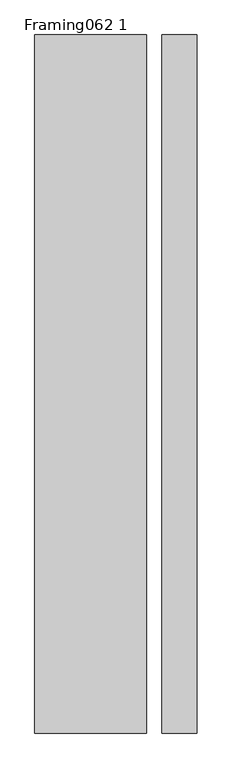
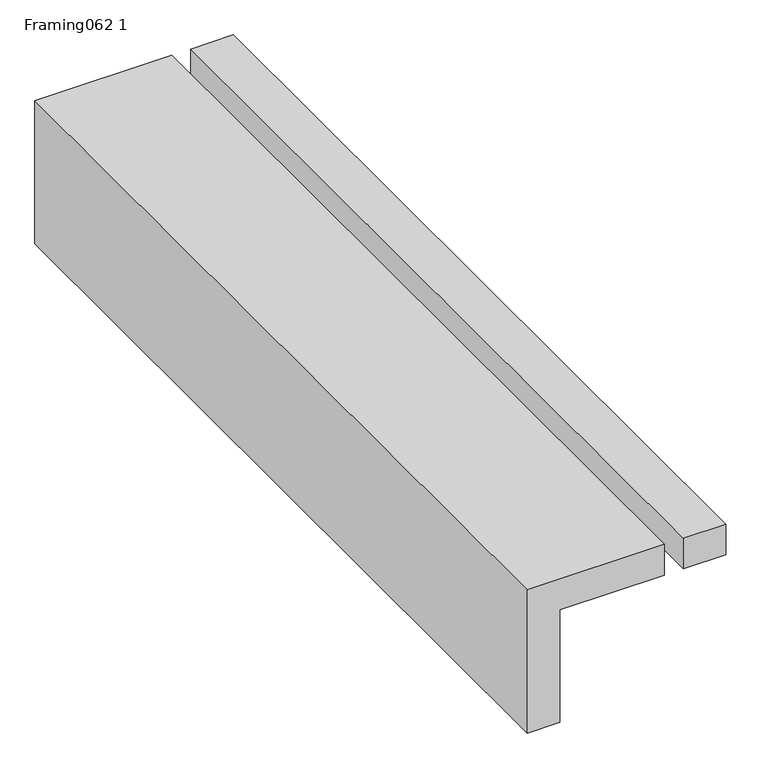
"""IFC4 building model written with IfcOpenShell, lengths in millimetres: proxy geometry, Framing062 1 : Framing062 15035."""

import ifcopenshell
import ifcopenshell.guid

model = None  # the IFC model being written
_history = None  # IfcOwnerHistory: only IFC2X3 demands one
_inside = {}  # id of a spatial element -> (the spatial element, [elements in it])
_under = {}  # id of a project, library or spatial element -> (it, [spatial elements below it])
_declared = {}  # id of a project -> (the project, [libraries it declares])
_typed = {}  # id of a type object -> (the type object, [elements of that type])
_made_of = {}  # id of a material, layer set ... -> (it, [elements and type objects made of it])


def new_model(schema):
    """Start an empty IFC model of exactly this schema.

    Asked for "IFC4X3", IfcOpenShell would pick the latest addendum, in which some entities
    have other attributes; the version numbers below select the first issue.
    IFC2X3 requires an IfcOwnerHistory on every rooted entity: one is made here for all.
    """
    global model, _history
    if schema == "IFC4X3":
        model = ifcopenshell.file(schema_version=(4, 3, 0, 0))
    else:
        model = ifcopenshell.file(schema=schema)
    _inside.clear()
    _under.clear()
    _declared.clear()
    _typed.clear()
    _made_of.clear()
    _history = None
    if model.schema == "IFC2X3":
        org = make("IfcOrganization", Name="unknown")
        user = make(
            "IfcPersonAndOrganization",
            ThePerson=make("IfcPerson", FamilyName="unknown"),
            TheOrganization=org,
        )
        app = make(
            "IfcApplication",
            ApplicationDeveloper=org,
            Version="unknown",
            ApplicationFullName="unknown",
            ApplicationIdentifier="unknown",
        )
        _history = make(
            "IfcOwnerHistory",
            OwningUser=user,
            OwningApplication=app,
            ChangeAction="ADDED",
            CreationDate=0,
        )
    return model


def make(cls, **values):
    """One entity of the class cls with the attributes given. An attribute that is None is left unset."""
    return model.create_entity(
        cls, **{name: value for name, value in values.items() if value is not None}
    )


def rooted(cls, **values):
    """An entity with a GlobalId (a new one), such as an element, a storey or a relation."""
    return make(cls, GlobalId=ifcopenshell.guid.new(), OwnerHistory=_history, **values)


def si_unit(unit_type, name, prefix=None):
    """IfcSIUnit, for example si_unit("LENGTHUNIT", "METRE", prefix="MILLI")."""
    return make("IfcSIUnit", UnitType=unit_type, Prefix=prefix, Name=name)


def assignment(units):
    """IfcUnitAssignment: the units of a project."""
    return None if units is None else make("IfcUnitAssignment", Units=units)


def point(xyz):
    """IfcCartesianPoint."""
    return None if xyz is None else make("IfcCartesianPoint", Coordinates=xyz)


def direction(xyz):
    """IfcDirection."""
    return None if xyz is None else make("IfcDirection", DirectionRatios=xyz)


def frame(location, z_axis=None, x_axis=None):
    """IfcAxis2Placement3D, a coordinate frame: its origin and axes. An axis left out is left unset."""
    return make(
        "IfcAxis2Placement3D",
        Location=point(location),
        Axis=direction(z_axis),
        RefDirection=direction(x_axis),
    )


def origin():
    """The frame at (0, 0, 0) with its axes left unset."""
    return frame((0.0, 0.0, 0.0))


def place(relative_to, where):
    """IfcLocalPlacement: puts the frame where relative to a parent placement (None: the world)."""
    return make(
        "IfcLocalPlacement", PlacementRelTo=relative_to, RelativePlacement=where
    )


def context(
    kind, dimensions, precision=None, world=None, true_north=None, identifier=None
):
    """IfcGeometricRepresentationContext, for example the 3D "Model" context."""
    return make(
        "IfcGeometricRepresentationContext",
        ContextIdentifier=identifier,
        ContextType=kind,
        CoordinateSpaceDimension=dimensions,
        Precision=precision,
        WorldCoordinateSystem=world,
        TrueNorth=true_north,
    )


def project(units=None, contexts=None):
    """IfcProject with its units and contexts."""
    return rooted(
        "IfcProject",
        Name="project",
        RepresentationContexts=contexts,
        UnitsInContext=assignment(units),
    )


def spatial(cls, under=None, at=None, **own):
    """A site, building, storey or space (cls), placed at a placement, below another one or the project."""
    s = rooted(cls, ObjectPlacement=at, **own)
    if under is not None:
        _under.setdefault(under.id(), (under, []))[1].append(s)
    return s


def polyline(points):
    """IfcPolyline through the points."""
    return make("IfcPolyline", Points=[point(p) for p in points])


def outline(outer, holes=None, kind="AREA"):
    """IfcArbitraryClosedProfileDef: a profile drawn as a closed curve; with holes, ...WithVoids."""
    if holes is None:
        return make("IfcArbitraryClosedProfileDef", ProfileType=kind, OuterCurve=outer)
    return make(
        "IfcArbitraryProfileDefWithVoids",
        ProfileType=kind,
        OuterCurve=outer,
        InnerCurves=holes,
    )


def extrude(swept, where, along, depth):
    """IfcExtrudedAreaSolid: the profile swept, set in the frame where, extruded along a direction by depth."""
    return make(
        "IfcExtrudedAreaSolid",
        SweptArea=swept,
        Position=where,
        ExtrudedDirection=direction(along),
        Depth=depth,
    )


def shape(context_of_items, identifier, shape_type, items):
    """IfcShapeRepresentation: the items that make up one representation, for example the "Body"."""
    return make(
        "IfcShapeRepresentation",
        ContextOfItems=context_of_items,
        RepresentationIdentifier=identifier,
        RepresentationType=shape_type,
        Items=items,
    )


def source(mapping_origin, context_of_items, identifier, shape_type, items):
    """IfcRepresentationMap: a shape defined once, which mapped items show again and again."""
    return make(
        "IfcRepresentationMap",
        MappingOrigin=mapping_origin,
        MappedRepresentation=shape(context_of_items, identifier, shape_type, items),
    )


def transform(
    local_origin,
    x_axis=None,
    y_axis=None,
    z_axis=None,
    scale=None,
    scale2=None,
    scale3=None,
    uniform=True,
):
    """IfcCartesianTransformationOperator3D, or its non-uniform kind. x_axis, y_axis, z_axis: its Axis1, 2, 3."""
    if uniform:
        return make(
            "IfcCartesianTransformationOperator3D",
            Axis1=direction(x_axis),
            Axis2=direction(y_axis),
            LocalOrigin=point(local_origin),
            Scale=scale,
            Axis3=direction(z_axis),
        )
    return make(
        "IfcCartesianTransformationOperator3DnonUniform",
        Axis1=direction(x_axis),
        Axis2=direction(y_axis),
        LocalOrigin=point(local_origin),
        Scale=scale,
        Axis3=direction(z_axis),
        Scale2=scale2,
        Scale3=scale3,
    )


def mapped(mapping_source, mapping_target):
    """IfcMappedItem: shows the shape of a source again, moved by a transform."""
    return make(
        "IfcMappedItem", MappingSource=mapping_source, MappingTarget=mapping_target
    )


def made_of(thing, what):
    """Note that an element or type object is made of a material, layer set ...; save() writes the relation."""
    if what is not None:
        _made_of.setdefault(what.id(), (what, []))[1].append(thing)
    return thing


def element(
    cls,
    number,
    at=None,
    inside=None,
    cuts=None,
    type_object=None,
    material=None,
    context=None,
    identifier="Body",
    shape_type=None,
    held_by="IfcProductDefinitionShape",
    body=None,
    shapes=None,
    **own,
):
    """One element of the class cls, such as IfcWall. Its Tag is "e" and its number.

    at: its placement. inside: the storey or other place that contains it. cuts: it is an
    opening in that element (IfcRelVoidsElement). A single representation is given by context,
    identifier, shape_type and body (its items); several are given by shapes. held_by: the class
    of the entity that holds the representations. save() writes the other relations.
    """
    e = rooted(cls, Tag="e%d" % number, ObjectPlacement=at, **own)
    if body is not None:
        shapes = [shape(context, identifier, shape_type, body)]
    if shapes is not None:
        e.Representation = make(held_by, Representations=shapes)
    if inside is not None:
        _inside.setdefault(inside.id(), (inside, []))[1].append(e)
    if cuts is not None:
        rooted(
            "IfcRelVoidsElement", RelatingBuildingElement=cuts, RelatedOpeningElement=e
        )
    if type_object is not None:
        _typed.setdefault(type_object.id(), (type_object, []))[1].append(e)
    return made_of(e, material)


def aggregate(whole, parts):
    """IfcRelAggregates: a whole, such as a stair, and the parts it consists of."""
    return rooted("IfcRelAggregates", RelatingObject=whole, RelatedObjects=parts)


def save(model, path):
    """Write the relations noted so far, then the file.

    IfcRelAggregates (storeys below a building ...), IfcRelContainedInSpatialStructure (elements
    in a storey), IfcRelDefinesByType, IfcRelAssociatesMaterial and IfcRelDeclares: one each for
    every whole, place, type object, material and project.
    """
    for whole, parts in _under.values():
        aggregate(whole, parts)
    for where, things in _inside.values():
        rooted(
            "IfcRelContainedInSpatialStructure",
            RelatedElements=things,
            RelatingStructure=where,
        )
    for kind, things in _typed.values():
        rooted("IfcRelDefinesByType", RelatedObjects=things, RelatingType=kind)
    for what, things in _made_of.values():
        rooted("IfcRelAssociatesMaterial", RelatedObjects=things, RelatingMaterial=what)
    for by, libraries in _declared.values():
        rooted("IfcRelDeclares", RelatingContext=by, RelatedDefinitions=libraries)
    model.write(path)


def framing062_1_cbcbbf25(model_context):
    return source(origin(), model_context, "Body", "SweptSolid", [
        extrude(outline(polyline([(42134.105552, -863.3885697), (42413.2036692, -863.3885697), (42413.2036692, -618.6019086), (42489.4036692, -618.6019086), (42489.4036692, -939.5885697), (42134.105552, -939.5885697), (42134.105552, -863.3885697)])), frame((0.0, -1052.8906574, 0.0), z_axis=(0.0, 1.0, 0.0), x_axis=(0.0, 0.0, 1.0)), (0.0, 0.0, 1.0), 2000.0),
        extrude(outline(polyline([(-474.2526923, -1052.8906574), (-574.1519086, -1052.8906574), (-574.1519086, 947.1093426), (-474.2526923, 947.1093426), (-474.2526923, -1052.8906574)])), frame((0.0, 0.0, 42413.2036692), z_axis=(0.0, 0.0, 1.0), x_axis=(1.0, 0.0, 0.0)), (0.0, 0.0, 1.0), 76.2),
    ])


if __name__ == "__main__":
    model = new_model("IFC4")
    model_context = context("Model", 3, world=origin())
    ifc_project = project(units=[si_unit("LENGTHUNIT", "METRE", prefix="MILLI")], contexts=[model_context])
    site = spatial("IfcSite", under=ifc_project)
    building = spatial("IfcBuilding", under=site)
    placement = place(None, origin())
    framing062_1_shape = framing062_1_cbcbbf25(model_context)
    element("IfcBuildingElementProxy", 1, Name="Framing062 1 : Framing062 15035", ObjectType="Framing062 1 : Framing062 15035", at=placement, inside=building, context=model_context, shape_type="MappedRepresentation", body=[
        mapped(framing062_1_shape, transform((0.0, 0.0, 0.0), x_axis=(1.0, 0.0, 0.0), y_axis=(0.0, 1.0, 0.0), z_axis=(0.0, 0.0, 1.0))),
    ])
    save(model, "model.ifc")

# Revit data of these elements
# Type "Framing062 1 : Framing062 15035"
#   NameOverride = "Framing062"
# Element 1 (IfcBuildingElementProxy, "Framing062 1 : Framing062 15035")
#   Materials on its faces: "POLYURETHANE SPRAY FOAM UNDER ROOF SUBSTRATE (SEE T-24 ENERGY REPORT FOR R-VALUE)"
# Materials
#   "POLYURETHANE SPRAY FOAM UNDER ROOF SUBSTRATE (SEE T-24 ENERGY REPORT FOR R-VALUE)": class "Unassigned", colour RGB 210 164 194, transparency 0, Cost = 0
